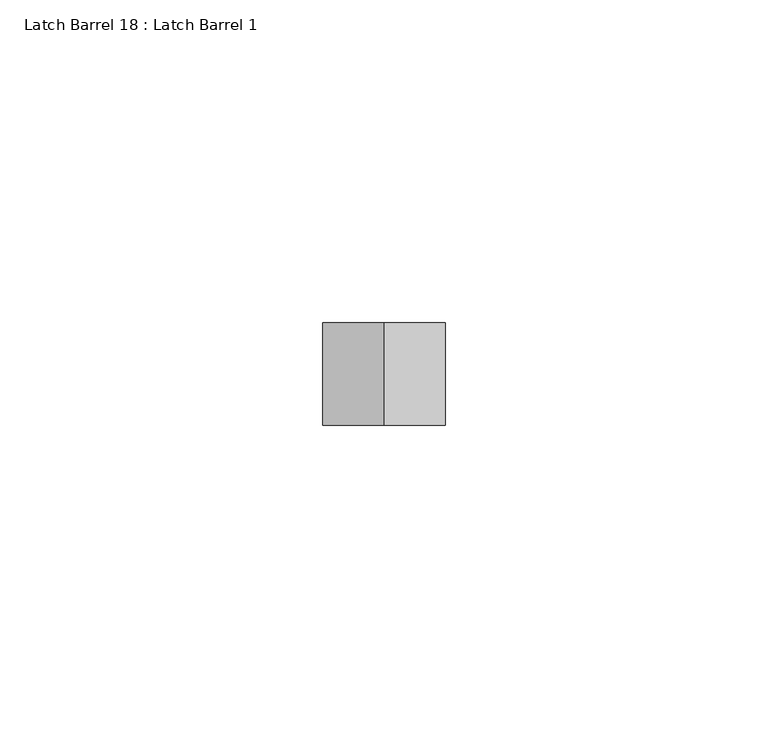
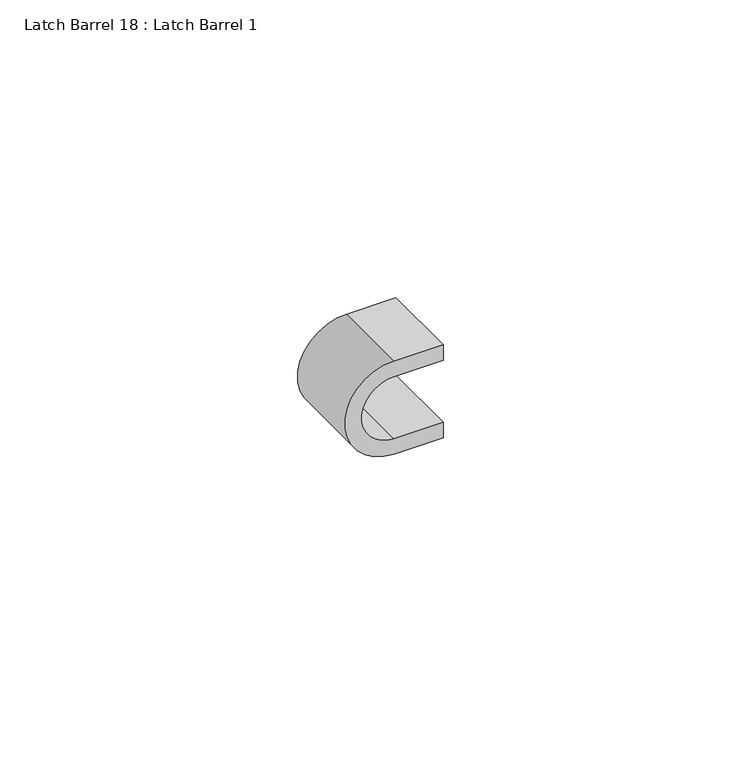
"""IFC4 building model written with IfcOpenShell, lengths in millimetres: proxy geometry, Latch Barrel 18 : Latch Barrel 1."""

from ifc_helpers import new_model, si_unit, point, frame, frame_2d, origin, place, context, project, spatial, polyline, circle_curve, trimmed, segment, composite_curve, outline, extrude, source, transform, mapped, element, save


def latch_barrel_18_latch_barrel_1_3a8c0b8a(model_context):
    return source(origin(), model_context, "Body", "SweptSolid", [
        extrude(outline(composite_curve([segment(trimmed(circle_curve(frame_2d((1066.8, 587312.7185739)), 6.35), [point((1060.45, 587312.7185739))], [point((1073.15, 587312.7185739))], True, "CARTESIAN"), True, "CONTINUOUS"), segment(polyline([(1073.15, 587312.7185739), (1073.15, 587322.2435739), (1076.325, 587322.2435739), (1076.325, 587312.7185739)]), True, "CONTINUOUS"), segment(trimmed(circle_curve(frame_2d((1066.8, 587312.7185739)), 9.525), [point((1076.325, 587312.7185739))], [point((1057.275, 587312.7185739))], False, "CARTESIAN"), True, "CONTINUOUS"), segment(polyline([(1057.275, 587312.7185739), (1057.275, 587322.2435739), (1060.45, 587322.2435739), (1060.45, 587312.7185739)]), True, "CONTINUOUS")], self_intersect=False)), frame((0.0, -535230.1413841, 0.0), z_axis=(0.0, 1.0, 0.0), x_axis=(0.0, 0.0, 1.0)), (0.0, 0.0, 1.0), 15.875),
    ])


if __name__ == "__main__":
    model = new_model("IFC4")
    model_context = context("Model", 3, world=origin())
    ifc_project = project(units=[si_unit("LENGTHUNIT", "METRE", prefix="MILLI")], contexts=[model_context])
    site = spatial("IfcSite", under=ifc_project)
    building = spatial("IfcBuilding", under=site)
    placement = place(None, origin())
    latch_barrel_18_latch_barrel_1_shape = latch_barrel_18_latch_barrel_1_3a8c0b8a(model_context)
    element("IfcBuildingElementProxy", 1, Name="Latch Barrel 18 : Latch Barrel 1", ObjectType="Latch Barrel 18 : Latch Barrel 1", at=placement, inside=building, context=model_context, shape_type="MappedRepresentation", body=[
        mapped(latch_barrel_18_latch_barrel_1_shape, transform((0.0, 0.0, 0.0), x_axis=(1.0, 0.0, 0.0), y_axis=(0.0, 1.0, 0.0), z_axis=(0.0, 0.0, 1.0))),
    ])
    save(model, "model.ifc")

# Revit data of these elements
# Element 1 (IfcBuildingElementProxy, "Latch Barrel 18 : Latch Barrel 1")
#   Materials on its faces: "GALV. GATE LATCH"
# Materials
#   "GALV. GATE LATCH": class "Metal", colour RGB 189 187 185, transparency 0, Description = "Carbon steel", Cost = 0
